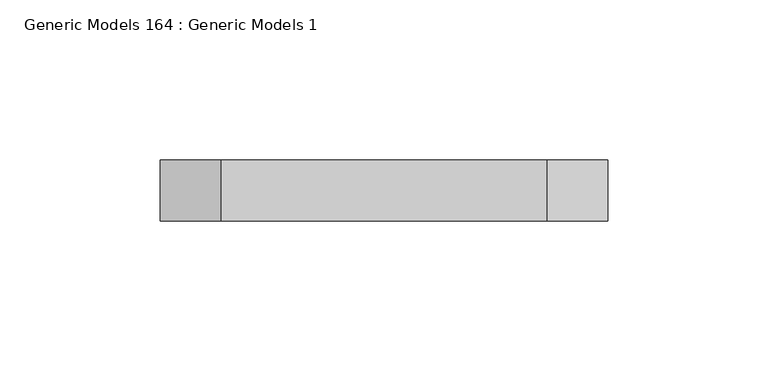
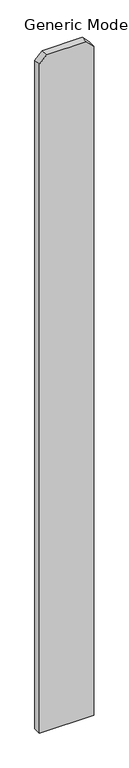
"""IFC4 building model written with IfcOpenShell, lengths in millimetres: proxy geometry, Generic Models 164 : Generic Models 1."""

import ifcopenshell
import ifcopenshell.guid

model = None  # the IFC model being written
_history = None  # IfcOwnerHistory: only IFC2X3 demands one
_inside = {}  # id of a spatial element -> (the spatial element, [elements in it])
_under = {}  # id of a project, library or spatial element -> (it, [spatial elements below it])
_declared = {}  # id of a project -> (the project, [libraries it declares])
_typed = {}  # id of a type object -> (the type object, [elements of that type])
_made_of = {}  # id of a material, layer set ... -> (it, [elements and type objects made of it])


def new_model(schema):
    """Start an empty IFC model of exactly this schema.

    Asked for "IFC4X3", IfcOpenShell would pick the latest addendum, in which some entities
    have other attributes; the version numbers below select the first issue.
    IFC2X3 requires an IfcOwnerHistory on every rooted entity: one is made here for all.
    """
    global model, _history
    if schema == "IFC4X3":
        model = ifcopenshell.file(schema_version=(4, 3, 0, 0))
    else:
        model = ifcopenshell.file(schema=schema)
    _inside.clear()
    _under.clear()
    _declared.clear()
    _typed.clear()
    _made_of.clear()
    _history = None
    if model.schema == "IFC2X3":
        org = make("IfcOrganization", Name="unknown")
        user = make(
            "IfcPersonAndOrganization",
            ThePerson=make("IfcPerson", FamilyName="unknown"),
            TheOrganization=org,
        )
        app = make(
            "IfcApplication",
            ApplicationDeveloper=org,
            Version="unknown",
            ApplicationFullName="unknown",
            ApplicationIdentifier="unknown",
        )
        _history = make(
            "IfcOwnerHistory",
            OwningUser=user,
            OwningApplication=app,
            ChangeAction="ADDED",
            CreationDate=0,
        )
    return model


def make(cls, **values):
    """One entity of the class cls with the attributes given. An attribute that is None is left unset."""
    return model.create_entity(
        cls, **{name: value for name, value in values.items() if value is not None}
    )


def rooted(cls, **values):
    """An entity with a GlobalId (a new one), such as an element, a storey or a relation."""
    return make(cls, GlobalId=ifcopenshell.guid.new(), OwnerHistory=_history, **values)


def si_unit(unit_type, name, prefix=None):
    """IfcSIUnit, for example si_unit("LENGTHUNIT", "METRE", prefix="MILLI")."""
    return make("IfcSIUnit", UnitType=unit_type, Prefix=prefix, Name=name)


def assignment(units):
    """IfcUnitAssignment: the units of a project."""
    return None if units is None else make("IfcUnitAssignment", Units=units)


def point(xyz):
    """IfcCartesianPoint."""
    return None if xyz is None else make("IfcCartesianPoint", Coordinates=xyz)


def direction(xyz):
    """IfcDirection."""
    return None if xyz is None else make("IfcDirection", DirectionRatios=xyz)


def frame(location, z_axis=None, x_axis=None):
    """IfcAxis2Placement3D, a coordinate frame: its origin and axes. An axis left out is left unset."""
    return make(
        "IfcAxis2Placement3D",
        Location=point(location),
        Axis=direction(z_axis),
        RefDirection=direction(x_axis),
    )


def origin():
    """The frame at (0, 0, 0) with its axes left unset."""
    return frame((0.0, 0.0, 0.0))


def place(relative_to, where):
    """IfcLocalPlacement: puts the frame where relative to a parent placement (None: the world)."""
    return make(
        "IfcLocalPlacement", PlacementRelTo=relative_to, RelativePlacement=where
    )


def context(
    kind, dimensions, precision=None, world=None, true_north=None, identifier=None
):
    """IfcGeometricRepresentationContext, for example the 3D "Model" context."""
    return make(
        "IfcGeometricRepresentationContext",
        ContextIdentifier=identifier,
        ContextType=kind,
        CoordinateSpaceDimension=dimensions,
        Precision=precision,
        WorldCoordinateSystem=world,
        TrueNorth=true_north,
    )


def project(units=None, contexts=None):
    """IfcProject with its units and contexts."""
    return rooted(
        "IfcProject",
        Name="project",
        RepresentationContexts=contexts,
        UnitsInContext=assignment(units),
    )


def spatial(cls, under=None, at=None, **own):
    """A site, building, storey or space (cls), placed at a placement, below another one or the project."""
    s = rooted(cls, ObjectPlacement=at, **own)
    if under is not None:
        _under.setdefault(under.id(), (under, []))[1].append(s)
    return s


def polyline(points):
    """IfcPolyline through the points."""
    return make("IfcPolyline", Points=[point(p) for p in points])


def outline(outer, holes=None, kind="AREA"):
    """IfcArbitraryClosedProfileDef: a profile drawn as a closed curve; with holes, ...WithVoids."""
    if holes is None:
        return make("IfcArbitraryClosedProfileDef", ProfileType=kind, OuterCurve=outer)
    return make(
        "IfcArbitraryProfileDefWithVoids",
        ProfileType=kind,
        OuterCurve=outer,
        InnerCurves=holes,
    )


def extrude(swept, where, along, depth):
    """IfcExtrudedAreaSolid: the profile swept, set in the frame where, extruded along a direction by depth."""
    return make(
        "IfcExtrudedAreaSolid",
        SweptArea=swept,
        Position=where,
        ExtrudedDirection=direction(along),
        Depth=depth,
    )


def shape(context_of_items, identifier, shape_type, items):
    """IfcShapeRepresentation: the items that make up one representation, for example the "Body"."""
    return make(
        "IfcShapeRepresentation",
        ContextOfItems=context_of_items,
        RepresentationIdentifier=identifier,
        RepresentationType=shape_type,
        Items=items,
    )


def source(mapping_origin, context_of_items, identifier, shape_type, items):
    """IfcRepresentationMap: a shape defined once, which mapped items show again and again."""
    return make(
        "IfcRepresentationMap",
        MappingOrigin=mapping_origin,
        MappedRepresentation=shape(context_of_items, identifier, shape_type, items),
    )


def transform(
    local_origin,
    x_axis=None,
    y_axis=None,
    z_axis=None,
    scale=None,
    scale2=None,
    scale3=None,
    uniform=True,
):
    """IfcCartesianTransformationOperator3D, or its non-uniform kind. x_axis, y_axis, z_axis: its Axis1, 2, 3."""
    if uniform:
        return make(
            "IfcCartesianTransformationOperator3D",
            Axis1=direction(x_axis),
            Axis2=direction(y_axis),
            LocalOrigin=point(local_origin),
            Scale=scale,
            Axis3=direction(z_axis),
        )
    return make(
        "IfcCartesianTransformationOperator3DnonUniform",
        Axis1=direction(x_axis),
        Axis2=direction(y_axis),
        LocalOrigin=point(local_origin),
        Scale=scale,
        Axis3=direction(z_axis),
        Scale2=scale2,
        Scale3=scale3,
    )


def mapped(mapping_source, mapping_target):
    """IfcMappedItem: shows the shape of a source again, moved by a transform."""
    return make(
        "IfcMappedItem", MappingSource=mapping_source, MappingTarget=mapping_target
    )


def made_of(thing, what):
    """Note that an element or type object is made of a material, layer set ...; save() writes the relation."""
    if what is not None:
        _made_of.setdefault(what.id(), (what, []))[1].append(thing)
    return thing


def element(
    cls,
    number,
    at=None,
    inside=None,
    cuts=None,
    type_object=None,
    material=None,
    context=None,
    identifier="Body",
    shape_type=None,
    held_by="IfcProductDefinitionShape",
    body=None,
    shapes=None,
    **own,
):
    """One element of the class cls, such as IfcWall. Its Tag is "e" and its number.

    at: its placement. inside: the storey or other place that contains it. cuts: it is an
    opening in that element (IfcRelVoidsElement). A single representation is given by context,
    identifier, shape_type and body (its items); several are given by shapes. held_by: the class
    of the entity that holds the representations. save() writes the other relations.
    """
    e = rooted(cls, Tag="e%d" % number, ObjectPlacement=at, **own)
    if body is not None:
        shapes = [shape(context, identifier, shape_type, body)]
    if shapes is not None:
        e.Representation = make(held_by, Representations=shapes)
    if inside is not None:
        _inside.setdefault(inside.id(), (inside, []))[1].append(e)
    if cuts is not None:
        rooted(
            "IfcRelVoidsElement", RelatingBuildingElement=cuts, RelatedOpeningElement=e
        )
    if type_object is not None:
        _typed.setdefault(type_object.id(), (type_object, []))[1].append(e)
    return made_of(e, material)


def aggregate(whole, parts):
    """IfcRelAggregates: a whole, such as a stair, and the parts it consists of."""
    return rooted("IfcRelAggregates", RelatingObject=whole, RelatedObjects=parts)


def save(model, path):
    """Write the relations noted so far, then the file.

    IfcRelAggregates (storeys below a building ...), IfcRelContainedInSpatialStructure (elements
    in a storey), IfcRelDefinesByType, IfcRelAssociatesMaterial and IfcRelDeclares: one each for
    every whole, place, type object, material and project.
    """
    for whole, parts in _under.values():
        aggregate(whole, parts)
    for where, things in _inside.values():
        rooted(
            "IfcRelContainedInSpatialStructure",
            RelatedElements=things,
            RelatingStructure=where,
        )
    for kind, things in _typed.values():
        rooted("IfcRelDefinesByType", RelatedObjects=things, RelatingType=kind)
    for what, things in _made_of.values():
        rooted("IfcRelAssociatesMaterial", RelatedObjects=things, RelatingMaterial=what)
    for by, libraries in _declared.values():
        rooted("IfcRelDeclares", RelatingContext=by, RelatedDefinitions=libraries)
    model.write(path)


def generic_models_164_generic_models_1_c75473e5(model_context):
    return source(origin(), model_context, "Body", "SweptSolid", [
        extrude(outline(polyline([(76.2, 54989.4125), (1885.95, 54989.4125), (1905.0, 54970.3625), (1905.0, 54868.7625), (1885.95, 54849.7125), (76.2, 54849.7125), (76.2, 54989.4125)])), frame((0.0, 547.6875, 0.0), z_axis=(0.0, 1.0, 0.0), x_axis=(0.0, 0.0, 1.0)), (0.0, 0.0, 1.0), 19.05),
    ])


if __name__ == "__main__":
    model = new_model("IFC4")
    model_context = context("Model", 3, world=origin())
    ifc_project = project(units=[si_unit("LENGTHUNIT", "METRE", prefix="MILLI")], contexts=[model_context])
    site = spatial("IfcSite", under=ifc_project)
    building = spatial("IfcBuilding", under=site)
    placement = place(None, origin())
    generic_models_164_generic_models_1_shape = generic_models_164_generic_models_1_c75473e5(model_context)
    element("IfcBuildingElementProxy", 1, Name="Generic Models 164 : Generic Models 1", ObjectType="Generic Models 164 : Generic Models 1", at=placement, inside=building, context=model_context, shape_type="MappedRepresentation", body=[
        mapped(generic_models_164_generic_models_1_shape, transform((0.0, 0.0, 0.0), x_axis=(1.0, 0.0, 0.0), y_axis=(0.0, 1.0, 0.0), z_axis=(0.0, 0.0, 1.0))),
    ])
    save(model, "model.ifc")

# Revit data of these elements
# Element 1 (IfcBuildingElementProxy, "Generic Models 164 : Generic Models 1")
#   Materials on its faces: "VERTICAL 1X6 CEDAR PLANKS W/ CLEAR WOOD SEALER"
# Materials
#   "VERTICAL 1X6 CEDAR PLANKS W/ CLEAR WOOD SEALER": class "Wood", colour RGB 234 198 147, transparency 0, Description = "Pinus Echinata", Cost = 0
